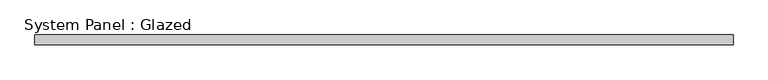
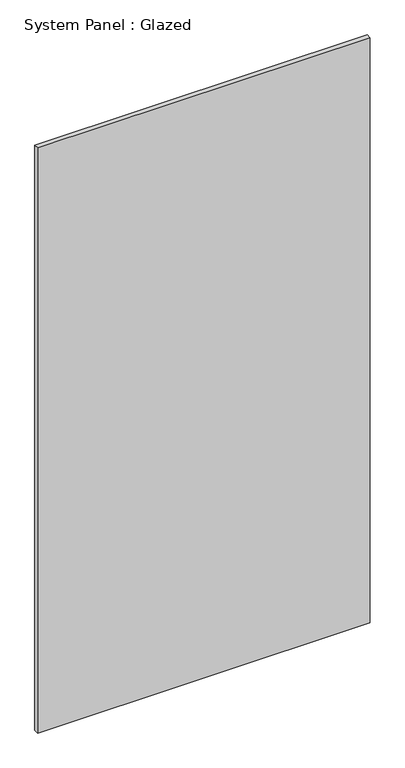
"""IFC4 building model written with IfcOpenShell, lengths in millimetres: plate geometry, System Panel : Glazed."""

import ifcopenshell
import ifcopenshell.guid

model = None  # the IFC model being written
_history = None  # IfcOwnerHistory: only IFC2X3 demands one
_inside = {}  # id of a spatial element -> (the spatial element, [elements in it])
_under = {}  # id of a project, library or spatial element -> (it, [spatial elements below it])
_declared = {}  # id of a project -> (the project, [libraries it declares])
_typed = {}  # id of a type object -> (the type object, [elements of that type])
_made_of = {}  # id of a material, layer set ... -> (it, [elements and type objects made of it])


def new_model(schema):
    """Start an empty IFC model of exactly this schema.

    Asked for "IFC4X3", IfcOpenShell would pick the latest addendum, in which some entities
    have other attributes; the version numbers below select the first issue.
    IFC2X3 requires an IfcOwnerHistory on every rooted entity: one is made here for all.
    """
    global model, _history
    if schema == "IFC4X3":
        model = ifcopenshell.file(schema_version=(4, 3, 0, 0))
    else:
        model = ifcopenshell.file(schema=schema)
    _inside.clear()
    _under.clear()
    _declared.clear()
    _typed.clear()
    _made_of.clear()
    _history = None
    if model.schema == "IFC2X3":
        org = make("IfcOrganization", Name="unknown")
        user = make(
            "IfcPersonAndOrganization",
            ThePerson=make("IfcPerson", FamilyName="unknown"),
            TheOrganization=org,
        )
        app = make(
            "IfcApplication",
            ApplicationDeveloper=org,
            Version="unknown",
            ApplicationFullName="unknown",
            ApplicationIdentifier="unknown",
        )
        _history = make(
            "IfcOwnerHistory",
            OwningUser=user,
            OwningApplication=app,
            ChangeAction="ADDED",
            CreationDate=0,
        )
    return model


def make(cls, **values):
    """One entity of the class cls with the attributes given. An attribute that is None is left unset."""
    return model.create_entity(
        cls, **{name: value for name, value in values.items() if value is not None}
    )


def rooted(cls, **values):
    """An entity with a GlobalId (a new one), such as an element, a storey or a relation."""
    return make(cls, GlobalId=ifcopenshell.guid.new(), OwnerHistory=_history, **values)


def si_unit(unit_type, name, prefix=None):
    """IfcSIUnit, for example si_unit("LENGTHUNIT", "METRE", prefix="MILLI")."""
    return make("IfcSIUnit", UnitType=unit_type, Prefix=prefix, Name=name)


def assignment(units):
    """IfcUnitAssignment: the units of a project."""
    return None if units is None else make("IfcUnitAssignment", Units=units)


def point(xyz):
    """IfcCartesianPoint."""
    return None if xyz is None else make("IfcCartesianPoint", Coordinates=xyz)


def direction(xyz):
    """IfcDirection."""
    return None if xyz is None else make("IfcDirection", DirectionRatios=xyz)


def frame(location, z_axis=None, x_axis=None):
    """IfcAxis2Placement3D, a coordinate frame: its origin and axes. An axis left out is left unset."""
    return make(
        "IfcAxis2Placement3D",
        Location=point(location),
        Axis=direction(z_axis),
        RefDirection=direction(x_axis),
    )


def origin():
    """The frame at (0, 0, 0) with its axes left unset."""
    return frame((0.0, 0.0, 0.0))


def origin_with_axes():
    """The frame at (0, 0, 0) with the z axis (0, 0, 1) and the x axis (1, 0, 0) written out."""
    return frame((0.0, 0.0, 0.0), z_axis=(0.0, 0.0, 1.0), x_axis=(1.0, 0.0, 0.0))


def place(relative_to, where):
    """IfcLocalPlacement: puts the frame where relative to a parent placement (None: the world)."""
    return make(
        "IfcLocalPlacement", PlacementRelTo=relative_to, RelativePlacement=where
    )


def context(
    kind, dimensions, precision=None, world=None, true_north=None, identifier=None
):
    """IfcGeometricRepresentationContext, for example the 3D "Model" context."""
    return make(
        "IfcGeometricRepresentationContext",
        ContextIdentifier=identifier,
        ContextType=kind,
        CoordinateSpaceDimension=dimensions,
        Precision=precision,
        WorldCoordinateSystem=world,
        TrueNorth=true_north,
    )


def project(units=None, contexts=None):
    """IfcProject with its units and contexts."""
    return rooted(
        "IfcProject",
        Name="project",
        RepresentationContexts=contexts,
        UnitsInContext=assignment(units),
    )


def spatial(cls, under=None, at=None, **own):
    """A site, building, storey or space (cls), placed at a placement, below another one or the project."""
    s = rooted(cls, ObjectPlacement=at, **own)
    if under is not None:
        _under.setdefault(under.id(), (under, []))[1].append(s)
    return s


def polyline(points):
    """IfcPolyline through the points."""
    return make("IfcPolyline", Points=[point(p) for p in points])


def outline(outer, holes=None, kind="AREA"):
    """IfcArbitraryClosedProfileDef: a profile drawn as a closed curve; with holes, ...WithVoids."""
    if holes is None:
        return make("IfcArbitraryClosedProfileDef", ProfileType=kind, OuterCurve=outer)
    return make(
        "IfcArbitraryProfileDefWithVoids",
        ProfileType=kind,
        OuterCurve=outer,
        InnerCurves=holes,
    )


def extrude(swept, where, along, depth):
    """IfcExtrudedAreaSolid: the profile swept, set in the frame where, extruded along a direction by depth."""
    return make(
        "IfcExtrudedAreaSolid",
        SweptArea=swept,
        Position=where,
        ExtrudedDirection=direction(along),
        Depth=depth,
    )


def shape(context_of_items, identifier, shape_type, items):
    """IfcShapeRepresentation: the items that make up one representation, for example the "Body"."""
    return make(
        "IfcShapeRepresentation",
        ContextOfItems=context_of_items,
        RepresentationIdentifier=identifier,
        RepresentationType=shape_type,
        Items=items,
    )


def source(mapping_origin, context_of_items, identifier, shape_type, items):
    """IfcRepresentationMap: a shape defined once, which mapped items show again and again."""
    return make(
        "IfcRepresentationMap",
        MappingOrigin=mapping_origin,
        MappedRepresentation=shape(context_of_items, identifier, shape_type, items),
    )


def transform(
    local_origin,
    x_axis=None,
    y_axis=None,
    z_axis=None,
    scale=None,
    scale2=None,
    scale3=None,
    uniform=True,
):
    """IfcCartesianTransformationOperator3D, or its non-uniform kind. x_axis, y_axis, z_axis: its Axis1, 2, 3."""
    if uniform:
        return make(
            "IfcCartesianTransformationOperator3D",
            Axis1=direction(x_axis),
            Axis2=direction(y_axis),
            LocalOrigin=point(local_origin),
            Scale=scale,
            Axis3=direction(z_axis),
        )
    return make(
        "IfcCartesianTransformationOperator3DnonUniform",
        Axis1=direction(x_axis),
        Axis2=direction(y_axis),
        LocalOrigin=point(local_origin),
        Scale=scale,
        Axis3=direction(z_axis),
        Scale2=scale2,
        Scale3=scale3,
    )


def mapped(mapping_source, mapping_target):
    """IfcMappedItem: shows the shape of a source again, moved by a transform."""
    return make(
        "IfcMappedItem", MappingSource=mapping_source, MappingTarget=mapping_target
    )


def made_of(thing, what):
    """Note that an element or type object is made of a material, layer set ...; save() writes the relation."""
    if what is not None:
        _made_of.setdefault(what.id(), (what, []))[1].append(thing)
    return thing


def element(
    cls,
    number,
    at=None,
    inside=None,
    cuts=None,
    type_object=None,
    material=None,
    context=None,
    identifier="Body",
    shape_type=None,
    held_by="IfcProductDefinitionShape",
    body=None,
    shapes=None,
    **own,
):
    """One element of the class cls, such as IfcWall. Its Tag is "e" and its number.

    at: its placement. inside: the storey or other place that contains it. cuts: it is an
    opening in that element (IfcRelVoidsElement). A single representation is given by context,
    identifier, shape_type and body (its items); several are given by shapes. held_by: the class
    of the entity that holds the representations. save() writes the other relations.
    """
    e = rooted(cls, Tag="e%d" % number, ObjectPlacement=at, **own)
    if body is not None:
        shapes = [shape(context, identifier, shape_type, body)]
    if shapes is not None:
        e.Representation = make(held_by, Representations=shapes)
    if inside is not None:
        _inside.setdefault(inside.id(), (inside, []))[1].append(e)
    if cuts is not None:
        rooted(
            "IfcRelVoidsElement", RelatingBuildingElement=cuts, RelatedOpeningElement=e
        )
    if type_object is not None:
        _typed.setdefault(type_object.id(), (type_object, []))[1].append(e)
    return made_of(e, material)


def aggregate(whole, parts):
    """IfcRelAggregates: a whole, such as a stair, and the parts it consists of."""
    return rooted("IfcRelAggregates", RelatingObject=whole, RelatedObjects=parts)


def save(model, path):
    """Write the relations noted so far, then the file.

    IfcRelAggregates (storeys below a building ...), IfcRelContainedInSpatialStructure (elements
    in a storey), IfcRelDefinesByType, IfcRelAssociatesMaterial and IfcRelDeclares: one each for
    every whole, place, type object, material and project.
    """
    for whole, parts in _under.values():
        aggregate(whole, parts)
    for where, things in _inside.values():
        rooted(
            "IfcRelContainedInSpatialStructure",
            RelatedElements=things,
            RelatingStructure=where,
        )
    for kind, things in _typed.values():
        rooted("IfcRelDefinesByType", RelatedObjects=things, RelatingType=kind)
    for what, things in _made_of.values():
        rooted("IfcRelAssociatesMaterial", RelatedObjects=things, RelatingMaterial=what)
    for by, libraries in _declared.values():
        rooted("IfcRelDeclares", RelatingContext=by, RelatedDefinitions=libraries)
    model.write(path)


def system_panel_glazed_6ec36b42(model_context):
    return source(origin(), model_context, "Body", "SweptSolid", [
        extrude(outline(polyline([(905.9413813, 24.5), (-905.9413813, 24.5), (-905.9413813, 49.5), (905.9413813, 49.5), (905.9413813, 24.5)])), origin_with_axes(), (0.0, 0.0, 1.0), 3370.0),
    ])


if __name__ == "__main__":
    model = new_model("IFC4")
    model_context = context("Model", 3, world=origin())
    ifc_project = project(units=[si_unit("LENGTHUNIT", "METRE", prefix="MILLI")], contexts=[model_context])
    site = spatial("IfcSite", under=ifc_project)
    building = spatial("IfcBuilding", under=site)
    placement = place(None, origin())
    system_panel_glazed_shape = system_panel_glazed_6ec36b42(model_context)
    element("IfcPlate", 1, ObjectType="System Panel : Glazed", at=placement, inside=building, context=model_context, shape_type="MappedRepresentation", body=[
        mapped(system_panel_glazed_shape, transform((0.0, 0.0, 0.0), x_axis=(1.0, 0.0, 0.0), y_axis=(0.0, 1.0, 0.0), z_axis=(0.0, 0.0, 1.0))),
    ])
    save(model, "model.ifc")

# Revit data of these elements
# Type "System Panel : Glazed"
#   Construction Type Id = "GSP4R"
#   Analytic Construction = "1/8 in Pilkington single glazing"
#   Visual Light Transmittance = 0.9
#   Solar Heat Gain Coefficient = 0.86
#   Heat Transfer Coefficient (U) = 6.7069 W/(m²·K)
#   Define Thermal Properties by = 1
# Element 1 (IfcPlate, "System Panel : Glazed")
#   Materials on its faces: "Glass"
# Materials
#   "Glass": class "Glass", colour RGB 245 245 243, transparency 1, Description = "Soda Lime Glass", Cost = 0
